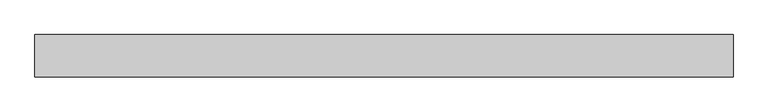
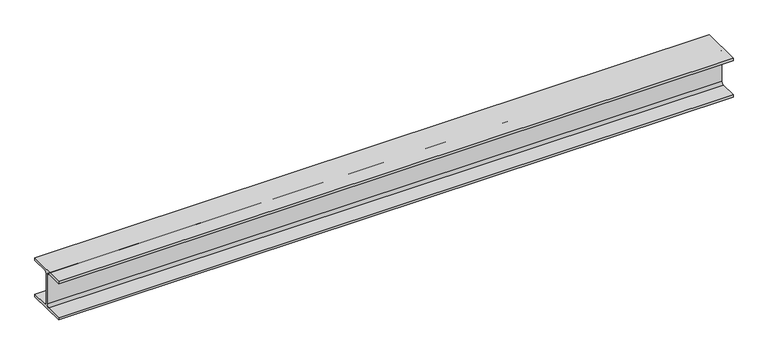
"""IFC4 building model written with IfcOpenShell, lengths in millimetres: beam geometry, 0912_Steel Framing_H-KSD3502 : H_SB_ASB_H-200x200x8x12."""

from ifc_helpers import new_model, si_unit, point, frame, frame_2d, origin, place, context, project, spatial, polyline, circle_curve, trimmed, segment, composite_curve, outline, extrude, source, transform, mapped, element, save


def beam_5ae02c5a(model_context):
    return source(origin(), model_context, "Body", "SweptSolid", [
        extrude(outline(composite_curve([segment(polyline([(100.0, -88.0), (100.0, -100.0), (-100.0, -100.0), (-100.0, -88.0), (-17.0, -88.0)]), True, "CONTINUOUS"), segment(trimmed(circle_curve(frame_2d((-17.0, -75.0)), 13.0), [point((-17.0, -88.0))], [point((-4.0, -75.0))], True, "CARTESIAN"), True, "CONTINUOUS"), segment(polyline([(-4.0, -75.0), (-4.0, 75.0)]), True, "CONTINUOUS"), segment(trimmed(circle_curve(frame_2d((-17.0, 75.0)), 13.0), [point((-4.0, 75.0))], [point((-17.0, 88.0))], True, "CARTESIAN"), True, "CONTINUOUS"), segment(polyline([(-17.0, 88.0), (-100.0, 88.0), (-100.0, 100.0), (100.0, 100.0), (100.0, 88.0), (17.0, 88.0)]), True, "CONTINUOUS"), segment(trimmed(circle_curve(frame_2d((17.0, 75.0)), 13.0), [point((17.0, 88.0))], [point((4.0, 75.0))], True, "CARTESIAN"), True, "CONTINUOUS"), segment(polyline([(4.0, 75.0), (4.0, -75.0)]), True, "CONTINUOUS"), segment(trimmed(circle_curve(frame_2d((17.0, -75.0)), 13.0), [point((4.0, -75.0))], [point((17.0, -88.0))], True, "CARTESIAN"), True, "CONTINUOUS"), segment(polyline([(17.0, -88.0), (100.0, -88.0)]), True, "CONTINUOUS")], self_intersect=False)), frame((-1700.2978834, 0.0, 0.0), z_axis=(1.0, 0.0, 0.0), x_axis=(0.0, 1.0, 0.0)), (0.0, 0.0, 1.0), 3294.9832404),
    ])


if __name__ == "__main__":
    model = new_model("IFC4")
    model_context = context("Model", 3, world=origin())
    ifc_project = project(units=[si_unit("LENGTHUNIT", "METRE", prefix="MILLI")], contexts=[model_context])
    site = spatial("IfcSite", under=ifc_project)
    building = spatial("IfcBuilding", under=site)
    placement = place(None, origin())
    beam_shape = beam_5ae02c5a(model_context)
    element("IfcBeam", 1, ObjectType="0912_Steel Framing_H-KSD3502 : H_SB_ASB_H-200x200x8x12", at=placement, inside=building, context=model_context, shape_type="MappedRepresentation", body=[
        mapped(beam_shape, transform((0.0, 0.0, 0.0), x_axis=(1.0, 0.0, 0.0), y_axis=(0.0, 1.0, 0.0), z_axis=(0.0, 0.0, 1.0))),
    ])
    save(model, "model.ifc")

# Revit data of these elements
# Type "0912_Steel Framing_H-KSD3502 : H_SB_ASB_H-200x200x8x12"
#   H_WM Code_1 = "S01AA002-00001 | Main Steel Structure Fabrication Work | Shelter/Building | Medium Steel - Standard (90KG/M>Weight≥30KG/M) | Material: (   )"
#   H_WM Code_2 = "S03AA028-00001 | Main Steel Structure Erection Work | Shelter/Building | Medium Steel (90KG/M>Weight≥30KG/M) | Material: (   )"
#   H_WM Code_3 = "S01AA010-00001 | Main Steel Structure Fabrication Work | Shelter/Building | Steel Painting/Coating | for Non-Fireproofed Steel Surface, Surface Preparation, Primer, Second & Final Coat | Material: (   )"
#   H_Q'ty Cal Type Tag = "SB-Q2"
#   Width = 20.0 cm
#   Web Thickness = 0.8 cm
#   Web Fillet = 1.3 cm
#   Warping Constant = 141000.0 cm⁶
#   W = 0
#   Torsional Moment of Inertia = 26.2485 cm⁴
#   Section Area = 63.53 cm²
#   Plastic Modulus weak axis = 244.0 cm³
#   Plastic Modulus strong axis = 525.0 cm³
#   Perimeter = 1.16 m²/m
#   Nominal Weight = 49.90 kgf/m
#   Moment of Inertia weak axis = 1600.00 cm⁴
#   Moment of Inertia strong axis = 4720.00 cm⁴
#   Height = 20.0 cm
#   Flange Thickness = 1.2 cm
#   Elastic Modulus weak axis = 160.0 cm³
#   Elastic Modulus strong axis = 472.0 cm³
#   Centroid Vertical = 10.0 cm
#   Centroid Horizontal = 10.0 cm
#   Ix = 47200000
#   Length [instance default] = 1.5240 m
#   Zx = 525000
#   b = 0.2000 m
#   h = 0.2000 m
#   r = 0.0130 m
#   s = 0.0080 m
#   t = 0.0120 m
#   A = 0.006353 m²
#   Structural Material [instance default] = Steel, 45-345
#   Assembly Code = ""
# Element 1 (IfcBeam, "0912_Steel Framing_H-KSD3502 : H_SB_ASB_H-200x200x8x12")
#   Structural Material = none
# Materials
#   "Steel, 45-345": class "Metal", colour RGB 189 187 185, transparency 0, Description = "Steel 345 MPa", Cost = 0
